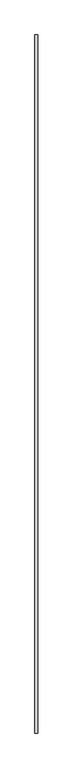
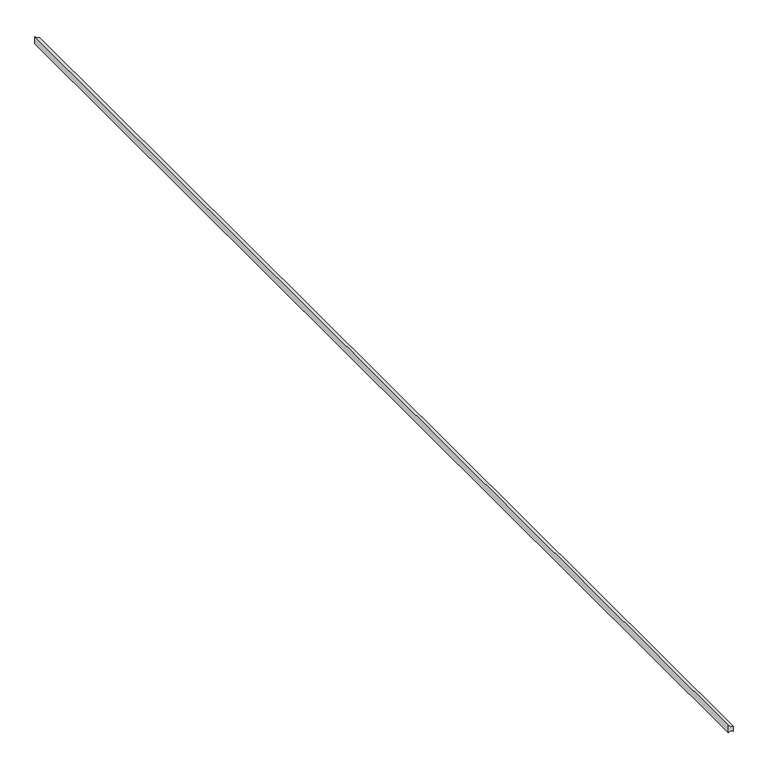
"""IFC4 building model written with IfcOpenShell, lengths in millimetres: proxy geometry, Joint048 8554 : Joint048 8554."""

from ifc_helpers import new_model, si_unit, point, frame, frame_2d, origin, place, context, project, spatial, polyline, circle_curve, trimmed, segment, composite_curve, outline, extrude, source, transform, mapped, element, save


def generic_models_285bbda0(model_context):
    return source(origin(), model_context, "Body", "SweptSolid", [
        extrude(outline(composite_curve([segment(polyline([(39560.2460083, -2103.2014185), (39568.2455813, -2103.2014185)]), True, "CONTINUOUS"), segment(trimmed(circle_curve(frame_2d((39578.8552996, -2102.2930179)), 10.6485359), [point((39568.2455813, -2103.2014185))], [point((39573.0722684, -2111.234375))], True, "CARTESIAN"), True, "CONTINUOUS"), segment(polyline([(39573.0722684, -2111.234375), (39560.2460083, -2111.234375)]), True, "CONTINUOUS"), segment(trimmed(circle_curve(frame_2d((39555.7238649, -2107.2178968)), 6.0482954), [point((39560.2460083, -2111.234375))], [point((39560.2460083, -2103.2014185))], True, "CARTESIAN"), True, "CONTINUOUS")], self_intersect=False)), frame((0.0, 998.1570038, 0.0), z_axis=(0.0, 1.0, 0.0), x_axis=(0.0, 0.0, 1.0)), (0.0, 0.0, 1.0), 2000.0),
    ])


if __name__ == "__main__":
    model = new_model("IFC4")
    model_context = context("Model", 3, world=origin())
    ifc_project = project(units=[si_unit("LENGTHUNIT", "METRE", prefix="MILLI")], contexts=[model_context])
    site = spatial("IfcSite", under=ifc_project)
    building = spatial("IfcBuilding", under=site)
    placement = place(None, origin())
    generic_models_shape = generic_models_285bbda0(model_context)
    element("IfcBuildingElementProxy", 1, Name="Joint048 8554 : Joint048 8554", ObjectType="Joint048 8554 : Joint048 8554", at=placement, inside=building, context=model_context, shape_type="MappedRepresentation", body=[
        mapped(generic_models_shape, transform((0.0, 0.0, 0.0), x_axis=(1.0, 0.0, 0.0), y_axis=(0.0, 1.0, 0.0), z_axis=(0.0, 0.0, 1.0))),
    ])
    save(model, "model.ifc")

# Revit data of these elements
# Type "Joint048 8554 : Joint048 8554"
#   NameOverride = "Joint048"
# Element 1 (IfcBuildingElementProxy, "Joint048 8554 : Joint048 8554")
#   Materials on its faces: "SEALANT"
# Materials
#   "SEALANT": class "Unassigned", colour RGB 142 225 148, transparency 0
